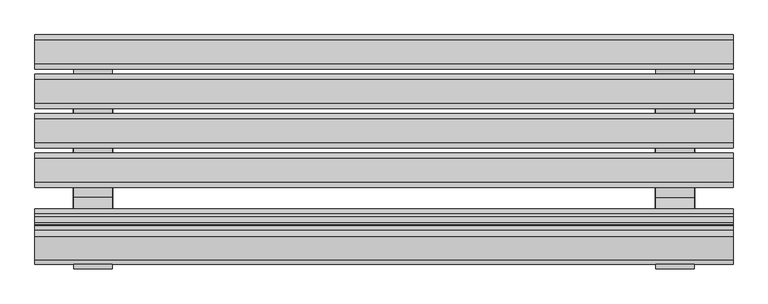
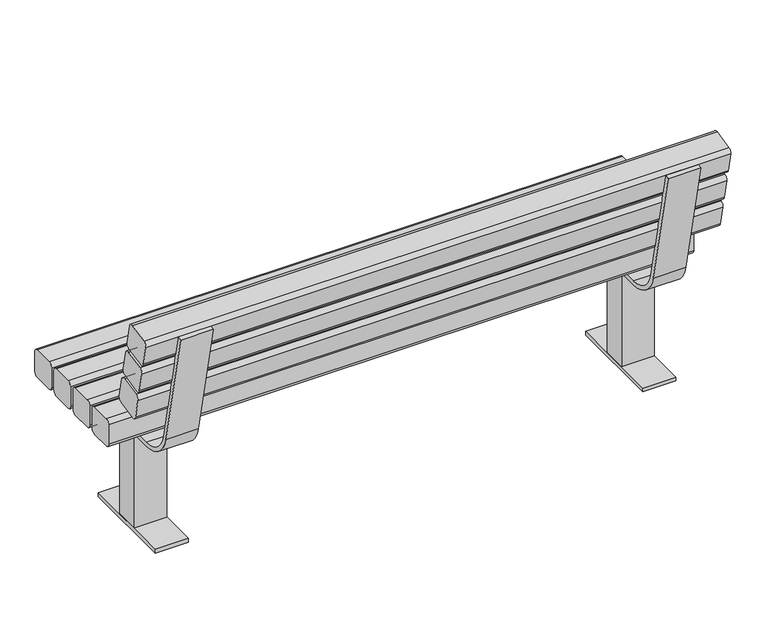
"""IFC4 building model written with IfcOpenShell, lengths in millimetres: furniture geometry, NLRS_90_FU_WPB_parkbank_gen_rsf : 1800mm breed."""

import ifcopenshell
import ifcopenshell.guid

model = None  # the IFC model being written
_history = None  # IfcOwnerHistory: only IFC2X3 demands one
_inside = {}  # id of a spatial element -> (the spatial element, [elements in it])
_under = {}  # id of a project, library or spatial element -> (it, [spatial elements below it])
_declared = {}  # id of a project -> (the project, [libraries it declares])
_typed = {}  # id of a type object -> (the type object, [elements of that type])
_made_of = {}  # id of a material, layer set ... -> (it, [elements and type objects made of it])


def new_model(schema):
    """Start an empty IFC model of exactly this schema.

    Asked for "IFC4X3", IfcOpenShell would pick the latest addendum, in which some entities
    have other attributes; the version numbers below select the first issue.
    IFC2X3 requires an IfcOwnerHistory on every rooted entity: one is made here for all.
    """
    global model, _history
    if schema == "IFC4X3":
        model = ifcopenshell.file(schema_version=(4, 3, 0, 0))
    else:
        model = ifcopenshell.file(schema=schema)
    _inside.clear()
    _under.clear()
    _declared.clear()
    _typed.clear()
    _made_of.clear()
    _history = None
    if model.schema == "IFC2X3":
        org = make("IfcOrganization", Name="unknown")
        user = make(
            "IfcPersonAndOrganization",
            ThePerson=make("IfcPerson", FamilyName="unknown"),
            TheOrganization=org,
        )
        app = make(
            "IfcApplication",
            ApplicationDeveloper=org,
            Version="unknown",
            ApplicationFullName="unknown",
            ApplicationIdentifier="unknown",
        )
        _history = make(
            "IfcOwnerHistory",
            OwningUser=user,
            OwningApplication=app,
            ChangeAction="ADDED",
            CreationDate=0,
        )
    return model


def make(cls, **values):
    """One entity of the class cls with the attributes given. An attribute that is None is left unset."""
    return model.create_entity(
        cls, **{name: value for name, value in values.items() if value is not None}
    )


def rooted(cls, **values):
    """An entity with a GlobalId (a new one), such as an element, a storey or a relation."""
    return make(cls, GlobalId=ifcopenshell.guid.new(), OwnerHistory=_history, **values)


def si_unit(unit_type, name, prefix=None):
    """IfcSIUnit, for example si_unit("LENGTHUNIT", "METRE", prefix="MILLI")."""
    return make("IfcSIUnit", UnitType=unit_type, Prefix=prefix, Name=name)


def assignment(units):
    """IfcUnitAssignment: the units of a project."""
    return None if units is None else make("IfcUnitAssignment", Units=units)


def point(xyz):
    """IfcCartesianPoint."""
    return None if xyz is None else make("IfcCartesianPoint", Coordinates=xyz)


def direction(xyz):
    """IfcDirection."""
    return None if xyz is None else make("IfcDirection", DirectionRatios=xyz)


def frame(location, z_axis=None, x_axis=None):
    """IfcAxis2Placement3D, a coordinate frame: its origin and axes. An axis left out is left unset."""
    return make(
        "IfcAxis2Placement3D",
        Location=point(location),
        Axis=direction(z_axis),
        RefDirection=direction(x_axis),
    )


def frame_2d(location, x_axis=None):
    """IfcAxis2Placement2D, a coordinate frame in the plane: its origin and x axis."""
    return make(
        "IfcAxis2Placement2D", Location=point(location), RefDirection=direction(x_axis)
    )


def origin():
    """The frame at (0, 0, 0) with its axes left unset."""
    return frame((0.0, 0.0, 0.0))


def origin_with_axes():
    """The frame at (0, 0, 0) with the z axis (0, 0, 1) and the x axis (1, 0, 0) written out."""
    return frame((0.0, 0.0, 0.0), z_axis=(0.0, 0.0, 1.0), x_axis=(1.0, 0.0, 0.0))


def place(relative_to, where):
    """IfcLocalPlacement: puts the frame where relative to a parent placement (None: the world)."""
    return make(
        "IfcLocalPlacement", PlacementRelTo=relative_to, RelativePlacement=where
    )


def context(
    kind, dimensions, precision=None, world=None, true_north=None, identifier=None
):
    """IfcGeometricRepresentationContext, for example the 3D "Model" context."""
    return make(
        "IfcGeometricRepresentationContext",
        ContextIdentifier=identifier,
        ContextType=kind,
        CoordinateSpaceDimension=dimensions,
        Precision=precision,
        WorldCoordinateSystem=world,
        TrueNorth=true_north,
    )


def project(units=None, contexts=None):
    """IfcProject with its units and contexts."""
    return rooted(
        "IfcProject",
        Name="project",
        RepresentationContexts=contexts,
        UnitsInContext=assignment(units),
    )


def spatial(cls, under=None, at=None, **own):
    """A site, building, storey or space (cls), placed at a placement, below another one or the project."""
    s = rooted(cls, ObjectPlacement=at, **own)
    if under is not None:
        _under.setdefault(under.id(), (under, []))[1].append(s)
    return s


def polyline(points):
    """IfcPolyline through the points."""
    return make("IfcPolyline", Points=[point(p) for p in points])


def circle_curve(where, radius):
    """IfcCircle in the frame where."""
    return make("IfcCircle", Position=where, Radius=radius)


def trimmed(basis, trim1, trim2, sense, master):
    """IfcTrimmedCurve: the piece of a basis curve between two trims."""
    return make(
        "IfcTrimmedCurve",
        BasisCurve=basis,
        Trim1=trim1,
        Trim2=trim2,
        SenseAgreement=sense,
        MasterRepresentation=master,
    )


def segment(curve, same_sense, transition):
    """IfcCompositeCurveSegment."""
    return make(
        "IfcCompositeCurveSegment",
        Transition=transition,
        SameSense=same_sense,
        ParentCurve=curve,
    )


def composite_curve(segments, self_intersect=None):
    """IfcCompositeCurve: segments joined end to end."""
    return make("IfcCompositeCurve", Segments=segments, SelfIntersect=self_intersect)


def outline(outer, holes=None, kind="AREA"):
    """IfcArbitraryClosedProfileDef: a profile drawn as a closed curve; with holes, ...WithVoids."""
    if holes is None:
        return make("IfcArbitraryClosedProfileDef", ProfileType=kind, OuterCurve=outer)
    return make(
        "IfcArbitraryProfileDefWithVoids",
        ProfileType=kind,
        OuterCurve=outer,
        InnerCurves=holes,
    )


def extrude(swept, where, along, depth):
    """IfcExtrudedAreaSolid: the profile swept, set in the frame where, extruded along a direction by depth."""
    return make(
        "IfcExtrudedAreaSolid",
        SweptArea=swept,
        Position=where,
        ExtrudedDirection=direction(along),
        Depth=depth,
    )


def shape(context_of_items, identifier, shape_type, items):
    """IfcShapeRepresentation: the items that make up one representation, for example the "Body"."""
    return make(
        "IfcShapeRepresentation",
        ContextOfItems=context_of_items,
        RepresentationIdentifier=identifier,
        RepresentationType=shape_type,
        Items=items,
    )


def source(mapping_origin, context_of_items, identifier, shape_type, items):
    """IfcRepresentationMap: a shape defined once, which mapped items show again and again."""
    return make(
        "IfcRepresentationMap",
        MappingOrigin=mapping_origin,
        MappedRepresentation=shape(context_of_items, identifier, shape_type, items),
    )


def transform(
    local_origin,
    x_axis=None,
    y_axis=None,
    z_axis=None,
    scale=None,
    scale2=None,
    scale3=None,
    uniform=True,
):
    """IfcCartesianTransformationOperator3D, or its non-uniform kind. x_axis, y_axis, z_axis: its Axis1, 2, 3."""
    if uniform:
        return make(
            "IfcCartesianTransformationOperator3D",
            Axis1=direction(x_axis),
            Axis2=direction(y_axis),
            LocalOrigin=point(local_origin),
            Scale=scale,
            Axis3=direction(z_axis),
        )
    return make(
        "IfcCartesianTransformationOperator3DnonUniform",
        Axis1=direction(x_axis),
        Axis2=direction(y_axis),
        LocalOrigin=point(local_origin),
        Scale=scale,
        Axis3=direction(z_axis),
        Scale2=scale2,
        Scale3=scale3,
    )


def mapped(mapping_source, mapping_target):
    """IfcMappedItem: shows the shape of a source again, moved by a transform."""
    return make(
        "IfcMappedItem", MappingSource=mapping_source, MappingTarget=mapping_target
    )


def made_of(thing, what):
    """Note that an element or type object is made of a material, layer set ...; save() writes the relation."""
    if what is not None:
        _made_of.setdefault(what.id(), (what, []))[1].append(thing)
    return thing


def element(
    cls,
    number,
    at=None,
    inside=None,
    cuts=None,
    type_object=None,
    material=None,
    context=None,
    identifier="Body",
    shape_type=None,
    held_by="IfcProductDefinitionShape",
    body=None,
    shapes=None,
    **own,
):
    """One element of the class cls, such as IfcWall. Its Tag is "e" and its number.

    at: its placement. inside: the storey or other place that contains it. cuts: it is an
    opening in that element (IfcRelVoidsElement). A single representation is given by context,
    identifier, shape_type and body (its items); several are given by shapes. held_by: the class
    of the entity that holds the representations. save() writes the other relations.
    """
    e = rooted(cls, Tag="e%d" % number, ObjectPlacement=at, **own)
    if body is not None:
        shapes = [shape(context, identifier, shape_type, body)]
    if shapes is not None:
        e.Representation = make(held_by, Representations=shapes)
    if inside is not None:
        _inside.setdefault(inside.id(), (inside, []))[1].append(e)
    if cuts is not None:
        rooted(
            "IfcRelVoidsElement", RelatingBuildingElement=cuts, RelatedOpeningElement=e
        )
    if type_object is not None:
        _typed.setdefault(type_object.id(), (type_object, []))[1].append(e)
    return made_of(e, material)


def aggregate(whole, parts):
    """IfcRelAggregates: a whole, such as a stair, and the parts it consists of."""
    return rooted("IfcRelAggregates", RelatingObject=whole, RelatedObjects=parts)


def save(model, path):
    """Write the relations noted so far, then the file.

    IfcRelAggregates (storeys below a building ...), IfcRelContainedInSpatialStructure (elements
    in a storey), IfcRelDefinesByType, IfcRelAssociatesMaterial and IfcRelDeclares: one each for
    every whole, place, type object, material and project.
    """
    for whole, parts in _under.values():
        aggregate(whole, parts)
    for where, things in _inside.values():
        rooted(
            "IfcRelContainedInSpatialStructure",
            RelatedElements=things,
            RelatingStructure=where,
        )
    for kind, things in _typed.values():
        rooted("IfcRelDefinesByType", RelatedObjects=things, RelatingType=kind)
    for what, things in _made_of.values():
        rooted("IfcRelAssociatesMaterial", RelatedObjects=things, RelatingMaterial=what)
    for by, libraries in _declared.values():
        rooted("IfcRelDeclares", RelatingContext=by, RelatedDefinitions=libraries)
    model.write(path)


def furniture_d88922e8(model_context):
    return source(origin(), model_context, "Body", "SweptSolid", [
        extrude(outline(polyline([(-778.4316018, 207.3631555), (-778.4316018, 512.1631555), (-676.8316018, 512.1631555), (-676.8316018, 207.3631555), (-778.4316018, 207.3631555)])), origin_with_axes(), (0.0, 0.0, 1.0), 12.7),
        extrude(outline(polyline([(722.3683982, 321.6631555), (722.3683982, 397.8631555), (822.3683982, 397.8631555), (822.3683982, 321.6631555), (722.3683982, 321.6631555)])), frame((0.0, 0.0, 12.7), z_axis=(0.0, 0.0, 1.0), x_axis=(1.0, 0.0, 0.0)), (0.0, 0.0, 1.0), 304.8),
        extrude(outline(composite_curve([segment(polyline([(85.9429731, 777.6296037), (165.0207138, 405.5980841)]), True, "CONTINUOUS"), segment(trimmed(circle_curve(frame_2d((258.1892727, 425.4016727)), 95.25), [point((165.0207138, 405.5980841))], [point((258.1892727, 330.1516727))], True, "CARTESIAN"), True, "CONTINUOUS"), segment(polyline([(258.1892727, 330.1516727), (656.6612098, 330.1516727), (656.6612098, 317.5), (258.1790004, 317.5)]), True, "CONTINUOUS"), segment(trimmed(circle_curve(frame_2d((258.1790004, 425.45)), 107.95), [point((258.1790004, 317.5))], [point((152.5879669, 403.005933))], False, "CARTESIAN"), True, "CONTINUOUS"), segment(polyline([(152.5879669, 403.005933), (73.5204986, 774.9891252), (85.9429731, 777.6296037)]), True, "CONTINUOUS")], self_intersect=False)), frame((722.3683982, 0.0, 0.0), z_axis=(1.0, 0.0, 0.0), x_axis=(0.0, 1.0, 0.0)), (0.0, 0.0, 1.0), 100.0),
        extrude(outline(polyline([(-677.6316018, 321.6631555), (-777.6316018, 321.6631555), (-777.6316018, 397.8631555), (-677.6316018, 397.8631555), (-677.6316018, 321.6631555)])), frame((0.0, 0.0, 12.7), z_axis=(0.0, 0.0, 1.0), x_axis=(1.0, 0.0, 0.0)), (0.0, 0.0, 1.0), 304.8),
        extrude(outline(polyline([(823.1683982, 207.3631555), (721.5683982, 207.3631555), (721.5683982, 512.1631555), (823.1683982, 512.1631555), (823.1683982, 207.3631555)])), origin_with_axes(), (0.0, 0.0, 1.0), 12.7),
        extrude(outline(composite_curve([segment(trimmed(circle_curve(frame_2d((202.7254759, 594.7128821)), 12.7), [point((200.0849974, 607.1353566))], [point((215.1479504, 597.3533605))], False, "CARTESIAN"), True, "CONTINUOUS"), segment(polyline([(215.1479504, 597.3533605), (228.3503428, 535.2409879)]), True, "CONTINUOUS"), segment(trimmed(circle_curve(frame_2d((215.9278683, 532.6005094)), 12.7), [point((228.3503428, 535.2409879))], [point((218.5683467, 520.1780349))], False, "CARTESIAN"), True, "CONTINUOUS"), segment(polyline([(218.5683467, 520.1780349), (156.4559741, 506.9756425)]), True, "CONTINUOUS"), segment(trimmed(circle_curve(frame_2d((153.8154956, 519.398117)), 12.7), [point((156.4559741, 506.9756425))], [point((141.3930211, 516.7576386))], False, "CARTESIAN"), True, "CONTINUOUS"), segment(polyline([(141.3930211, 516.7576386), (128.1906287, 578.8700112)]), True, "CONTINUOUS"), segment(trimmed(circle_curve(frame_2d((140.6131032, 581.5104897)), 12.7), [point((128.1906287, 578.8700112))], [point((137.9726248, 593.9329642))], False, "CARTESIAN"), True, "CONTINUOUS"), segment(polyline([(137.9726248, 593.9329642), (200.0849974, 607.1353566)]), True, "CONTINUOUS")], self_intersect=False)), frame((-877.6316018, 0.0, 0.0), z_axis=(1.0, 0.0, 0.0), x_axis=(0.0, 1.0, 0.0)), (0.0, 0.0, 1.0), 1800.0),
        extrude(outline(composite_curve([segment(trimmed(circle_curve(frame_2d((181.6016481, 694.0926783)), 12.7), [point((178.9611696, 706.5151528))], [point((194.0241226, 696.7331568))], False, "CARTESIAN"), True, "CONTINUOUS"), segment(polyline([(194.0241226, 696.7331568), (207.226515, 634.6207841)]), True, "CONTINUOUS"), segment(trimmed(circle_curve(frame_2d((194.8040405, 631.9803056)), 12.7), [point((207.226515, 634.6207841))], [point((197.4445189, 619.5578311))], False, "CARTESIAN"), True, "CONTINUOUS"), segment(polyline([(197.4445189, 619.5578311), (135.3321463, 606.3554388)]), True, "CONTINUOUS"), segment(trimmed(circle_curve(frame_2d((132.6916678, 618.7779133)), 12.7), [point((135.3321463, 606.3554388))], [point((120.2691933, 616.1374348))], False, "CARTESIAN"), True, "CONTINUOUS"), segment(polyline([(120.2691933, 616.1374348), (107.0668009, 678.2498075)]), True, "CONTINUOUS"), segment(trimmed(circle_curve(frame_2d((119.4892755, 680.8902859)), 12.7), [point((107.0668009, 678.2498075))], [point((116.848797, 693.3127605))], False, "CARTESIAN"), True, "CONTINUOUS"), segment(polyline([(116.848797, 693.3127605), (178.9611696, 706.5151528)]), True, "CONTINUOUS")], self_intersect=False)), frame((-877.6316018, 0.0, 0.0), z_axis=(1.0, 0.0, 0.0), x_axis=(0.0, 1.0, 0.0)), (0.0, 0.0, 1.0), 1800.0),
        extrude(outline(composite_curve([segment(polyline([(85.9429731, 777.6296037), (165.0207138, 405.5980841)]), True, "CONTINUOUS"), segment(trimmed(circle_curve(frame_2d((258.1892727, 425.4016727)), 95.25), [point((165.0207138, 405.5980841))], [point((258.1892727, 330.1516727))], True, "CARTESIAN"), True, "CONTINUOUS"), segment(polyline([(258.1892727, 330.1516727), (656.6612098, 330.1516727), (656.6612098, 317.5), (258.1790004, 317.5)]), True, "CONTINUOUS"), segment(trimmed(circle_curve(frame_2d((258.1790004, 425.45)), 107.95), [point((258.1790004, 317.5))], [point((152.5879669, 403.005933))], False, "CARTESIAN"), True, "CONTINUOUS"), segment(polyline([(152.5879669, 403.005933), (73.5204986, 774.9891252), (85.9429731, 777.6296037)]), True, "CONTINUOUS")], self_intersect=False)), frame((-777.6316018, 0.0, 0.0), z_axis=(1.0, 0.0, 0.0), x_axis=(0.0, 1.0, 0.0)), (0.0, 0.0, 1.0), 100.0),
        extrude(outline(composite_curve([segment(trimmed(circle_curve(frame_2d((160.4778203, 793.4724745)), 12.7), [point((157.8373418, 805.8949491))], [point((172.9002948, 796.112953))], False, "CARTESIAN"), True, "CONTINUOUS"), segment(polyline([(172.9002948, 796.112953), (186.1026872, 734.0005804)]), True, "CONTINUOUS"), segment(trimmed(circle_curve(frame_2d((173.6802127, 731.3601019)), 12.7), [point((186.1026872, 734.0005804))], [point((176.3206912, 718.9376274))], False, "CARTESIAN"), True, "CONTINUOUS"), segment(polyline([(176.3206912, 718.9376274), (114.2083185, 705.735235)]), True, "CONTINUOUS"), segment(trimmed(circle_curve(frame_2d((111.56784, 718.1577095)), 12.7), [point((114.2083185, 705.735235))], [point((99.1453655, 715.517231))], False, "CARTESIAN"), True, "CONTINUOUS"), segment(polyline([(99.1453655, 715.517231), (85.9429731, 777.6296037)]), True, "CONTINUOUS"), segment(trimmed(circle_curve(frame_2d((98.3654477, 780.2700822)), 12.7), [point((85.9429731, 777.6296037))], [point((95.7249692, 792.6925567))], False, "CARTESIAN"), True, "CONTINUOUS"), segment(polyline([(95.7249692, 792.6925567), (157.8373418, 805.8949491)]), True, "CONTINUOUS")], self_intersect=False)), frame((-877.6316018, 0.0, 0.0), z_axis=(1.0, 0.0, 0.0), x_axis=(0.0, 1.0, 0.0)), (0.0, 0.0, 1.0), 1800.0),
        extrude(outline(composite_curve([segment(trimmed(circle_curve(frame_2d((665.0298429, 406.3516727)), 12.7), [point((665.0298429, 419.0516727))], [point((677.7298429, 406.3516727))], False, "CARTESIAN"), True, "CONTINUOUS"), segment(polyline([(677.7298429, 406.3516727), (677.7298429, 342.8516727)]), True, "CONTINUOUS"), segment(trimmed(circle_curve(frame_2d((665.0298429, 342.8516727)), 12.7), [point((677.7298429, 342.8516727))], [point((665.0298429, 330.1516727))], False, "CARTESIAN"), True, "CONTINUOUS"), segment(polyline([(665.0298429, 330.1516727), (601.5298429, 330.1516727)]), True, "CONTINUOUS"), segment(trimmed(circle_curve(frame_2d((601.5298429, 342.8516727)), 12.7), [point((601.5298429, 330.1516727))], [point((588.8298429, 342.8516727))], False, "CARTESIAN"), True, "CONTINUOUS"), segment(polyline([(588.8298429, 342.8516727), (588.8298429, 406.3516727)]), True, "CONTINUOUS"), segment(trimmed(circle_curve(frame_2d((601.5298429, 406.3516727)), 12.7), [point((588.8298429, 406.3516727))], [point((601.5298429, 419.0516727))], False, "CARTESIAN"), True, "CONTINUOUS"), segment(polyline([(601.5298429, 419.0516727), (665.0298429, 419.0516727)]), True, "CONTINUOUS")], self_intersect=False)), frame((-877.6316018, 0.0, 0.0), z_axis=(1.0, 0.0, 0.0), x_axis=(0.0, 1.0, 0.0)), (0.0, 0.0, 1.0), 1800.0),
        extrude(outline(composite_curve([segment(trimmed(circle_curve(frame_2d((563.4298429, 406.3516727)), 12.7), [point((563.4298429, 419.0516727))], [point((576.1298429, 406.3516727))], False, "CARTESIAN"), True, "CONTINUOUS"), segment(polyline([(576.1298429, 406.3516727), (576.1298429, 342.8516727)]), True, "CONTINUOUS"), segment(trimmed(circle_curve(frame_2d((563.4298429, 342.8516727)), 12.7), [point((576.1298429, 342.8516727))], [point((563.4298429, 330.1516727))], False, "CARTESIAN"), True, "CONTINUOUS"), segment(polyline([(563.4298429, 330.1516727), (499.9298429, 330.1516727)]), True, "CONTINUOUS"), segment(trimmed(circle_curve(frame_2d((499.9298429, 342.8516727)), 12.7), [point((499.9298429, 330.1516727))], [point((487.2298429, 342.8516727))], False, "CARTESIAN"), True, "CONTINUOUS"), segment(polyline([(487.2298429, 342.8516727), (487.2298429, 406.3516727)]), True, "CONTINUOUS"), segment(trimmed(circle_curve(frame_2d((499.9298429, 406.3516727)), 12.7), [point((487.2298429, 406.3516727))], [point((499.9298429, 419.0516727))], False, "CARTESIAN"), True, "CONTINUOUS"), segment(polyline([(499.9298429, 419.0516727), (563.4298429, 419.0516727)]), True, "CONTINUOUS")], self_intersect=False)), frame((-877.6316018, 0.0, 0.0), z_axis=(1.0, 0.0, 0.0), x_axis=(0.0, 1.0, 0.0)), (0.0, 0.0, 1.0), 1800.0),
        extrude(outline(composite_curve([segment(trimmed(circle_curve(frame_2d((461.8298429, 406.3516727)), 12.7), [point((461.8298429, 419.0516727))], [point((474.5298429, 406.3516727))], False, "CARTESIAN"), True, "CONTINUOUS"), segment(polyline([(474.5298429, 406.3516727), (474.5298429, 342.8516727)]), True, "CONTINUOUS"), segment(trimmed(circle_curve(frame_2d((461.8298429, 342.8516727)), 12.7), [point((474.5298429, 342.8516727))], [point((461.8298429, 330.1516727))], False, "CARTESIAN"), True, "CONTINUOUS"), segment(polyline([(461.8298429, 330.1516727), (398.3298429, 330.1516727)]), True, "CONTINUOUS"), segment(trimmed(circle_curve(frame_2d((398.3298429, 342.8516727)), 12.7), [point((398.3298429, 330.1516727))], [point((385.6298429, 342.8516727))], False, "CARTESIAN"), True, "CONTINUOUS"), segment(polyline([(385.6298429, 342.8516727), (385.6298429, 406.3516727)]), True, "CONTINUOUS"), segment(trimmed(circle_curve(frame_2d((398.3298429, 406.3516727)), 12.7), [point((385.6298429, 406.3516727))], [point((398.3298429, 419.0516727))], False, "CARTESIAN"), True, "CONTINUOUS"), segment(polyline([(398.3298429, 419.0516727), (461.8298429, 419.0516727)]), True, "CONTINUOUS")], self_intersect=False)), frame((-877.6316018, 0.0, 0.0), z_axis=(1.0, 0.0, 0.0), x_axis=(0.0, 1.0, 0.0)), (0.0, 0.0, 1.0), 1800.0),
        extrude(outline(composite_curve([segment(trimmed(circle_curve(frame_2d((360.2298429, 406.3516727)), 12.7), [point((360.2298429, 419.0516727))], [point((372.9298429, 406.3516727))], False, "CARTESIAN"), True, "CONTINUOUS"), segment(polyline([(372.9298429, 406.3516727), (372.9298429, 342.8516727)]), True, "CONTINUOUS"), segment(trimmed(circle_curve(frame_2d((360.2298429, 342.8516727)), 12.7), [point((372.9298429, 342.8516727))], [point((360.2298429, 330.1516727))], False, "CARTESIAN"), True, "CONTINUOUS"), segment(polyline([(360.2298429, 330.1516727), (296.7298429, 330.1516727)]), True, "CONTINUOUS"), segment(trimmed(circle_curve(frame_2d((296.7298429, 342.8516727)), 12.7), [point((296.7298429, 330.1516727))], [point((284.0298429, 342.8516727))], False, "CARTESIAN"), True, "CONTINUOUS"), segment(polyline([(284.0298429, 342.8516727), (284.0298429, 406.3516727)]), True, "CONTINUOUS"), segment(trimmed(circle_curve(frame_2d((296.7298429, 406.3516727)), 12.7), [point((284.0298429, 406.3516727))], [point((296.7298429, 419.0516727))], False, "CARTESIAN"), True, "CONTINUOUS"), segment(polyline([(296.7298429, 419.0516727), (360.2298429, 419.0516727)]), True, "CONTINUOUS")], self_intersect=False)), frame((-877.6316018, 0.0, 0.0), z_axis=(1.0, 0.0, 0.0), x_axis=(0.0, 1.0, 0.0)), (0.0, 0.0, 1.0), 1800.0),
    ])


if __name__ == "__main__":
    model = new_model("IFC4")
    model_context = context("Model", 3, world=origin())
    ifc_project = project(units=[si_unit("LENGTHUNIT", "METRE", prefix="MILLI")], contexts=[model_context])
    site = spatial("IfcSite", under=ifc_project)
    building = spatial("IfcBuilding", under=site)
    placement = place(None, origin())
    furniture_shape = furniture_d88922e8(model_context)
    element("IfcFurniture", 1, ObjectType="NLRS_90_FU_WPB_parkbank_gen_rsf : 1800mm breed", at=placement, inside=building, context=model_context, shape_type="MappedRepresentation", body=[
        mapped(furniture_shape, transform((0.0, 0.0, 0.0), x_axis=(1.0, 0.0, 0.0), y_axis=(0.0, 1.0, 0.0), z_axis=(0.0, 0.0, 1.0))),
    ])
    save(model, "model.ifc")

# Revit data of these elements
# Type "NLRS_90_FU_WPB_parkbank_gen_rsf : 1800mm breed"
#   Type IFC Predefined Type = "USERDEFINED"
#   Export Type to IFC As = "IfcGeographicElementType"
#   Type IfcGUID = "05J6pyYiTDtR2exmlhyPly"
#   IfcName[Type] = "parkbank 1800mm breed"
#   IfcDescription[Type] = "parkbank b 1800mm"
#   IfcObjectType[Type] = "BENCH"
#   NLRS_C_revit_versie = ""
#   NLRS_C_omschrijving_02 = "onderstel"
#   NLRS_C_omschrijving_01 = "zitting"
#   NLRS_C_content_versie = ""
#   NLRS_C_content_provider = ""
#   NLRS_C_content_handleiding = ""
#   NLRS_C_content_datum_uitgifte = ""
#   NLRS_C_content_datum_gewijzigd = ""
#   NLRS_C_content_creator = ""
#   Model = "generiek"
#   Manufacturer = "Revit Standards Foundation"
#   Description = "parkbank b 1800mm"
#   Assembly Code = "90.71"
#   bf_overstek = 150.00 mm
#   NLRS_C_hoogte_01 [instance default] = 419.052 mm
#   NLRS_C_hoogte [instance default] = 806.45 mm
#   NLRS_C_diepte_01 [instance default] = 372.631 mm
#   NLRS_C_breedte = 1800.00 mm
#   Default Elevation = 1219.20 mm
#   NLRS_C_materiaal_02 = NLRS_h2_staal mat gepolijst grijs_gen_rsf
#   NLRS_C_materiaal_01 = NLRS_i3_hout loofhout meranti vernis_gen_rsf
# Element 1 (IfcFurniture, "NLRS_90_FU_WPB_parkbank_gen_rsf : 1800mm breed")
#   Materials on its faces: "NLRS_i3_hout loofhout meranti vernis_gen_rsf", "NLRS_h2_staal mat gepolijst grijs_gen_rsf"
# Materials
#   "NLRS_h2_staal mat gepolijst grijs_gen_rsf": class "System", colour RGB 189 187 185, transparency 0, Keynote = "h2", Model = "generiek", Manufacturer = "Revit Standards Foundation", URL = "www.revitstandards.org", Description = "staal mat gepolijst", Cost = 0
#   "NLRS_i3_hout loofhout meranti vernis_gen_rsf": class "Unassigned", colour RGB 227 170 128, transparency 0, Keynote = "i3", Model = "generiek", Manufacturer = "Revit Standards Foundation", URL = "www.revitstandards.org", Description = "loofhout merantie vernis", Cost = 0
